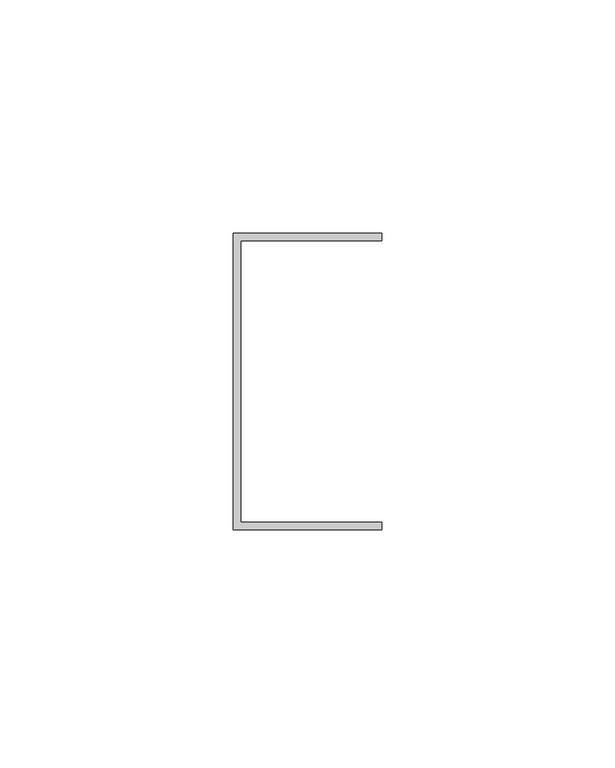
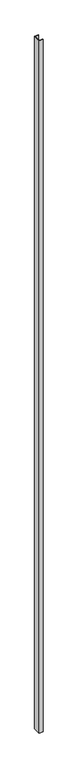
"""IFC4 building model written with IfcOpenShell, lengths in millimetres: proxy geometry, Generic Models 7:Generic Models 1:3:Generic Models 1:3 : Generic Models 7:Generic Models 1:305549:3:Generic Models 1:3:Generic Models 1:3 : Generic Models 7:Generic Models 1:305549:3 : Generic Models 7:Generic Models 1:3:Generic Models 1:3 : Generic Models 7:Generic Models 1:305549:301244:5 : Generic Models 7:Generic Models 1:3:Generic Models 1:3 : Generic Models 7:Generic Models 1:305549:3:Generic Models 1:3:Generic Models 1:3 : Generic Models 7:Generic Models 1:305549:3 : Generic Models 7:Generic Models 1:3:Generic Models 1:3 : Generic Models 7:Generic Models 1:305549:301244:308848."""

from ifc_helpers import new_model, si_unit, frame, origin, place, context, project, spatial, polyline, outline, extrude, source, transform, mapped, element, save


def generic_models_71cab8bc(model_context):
    return source(origin(), model_context, "Body", "SweptSolid", [
        extrude(outline(polyline([(570458.9867239, -579013.3913841), (570490.7367239, -579013.3913841), (570490.7367239, -579014.9788841), (570460.5742239, -579014.9788841), (570460.5742239, -579075.3038841), (570490.7367239, -579075.3038841), (570490.7367239, -579076.8913841), (570458.9867239, -579076.8913841), (570458.9867239, -579013.3913841)])), frame((0.0, 0.0, 38.1), z_axis=(0.0, 0.0, 1.0), x_axis=(1.0, 0.0, 0.0)), (0.0, 0.0, 1.0), 6096.0),
    ])


if __name__ == "__main__":
    model = new_model("IFC4")
    model_context = context("Model", 3, world=origin())
    ifc_project = project(units=[si_unit("LENGTHUNIT", "METRE", prefix="MILLI")], contexts=[model_context])
    site = spatial("IfcSite", under=ifc_project)
    building = spatial("IfcBuilding", under=site)
    placement = place(None, origin())
    generic_models_shape = generic_models_71cab8bc(model_context)
    element("IfcBuildingElementProxy", 1, Name="Generic Models 7:Generic Models 1:3:Generic Models 1:3 : Generic Models 7:Generic Models 1:305549:3:Generic Models 1:3:Generic Models 1:3 : Generic Models 7:Generic Models 1:305549:3 : Generic Models 7:Generic Models 1:3:Generic Models 1:3 : Generic Models 7:Generic Models 1:305549:301244:5 : Generic Models 7:Generic Models 1:3:Generic Models 1:3 : Generic Models 7:Generic Models 1:305549:3:Generic Models 1:3:Generic Models 1:3 : Generic Models 7:Generic Models 1:305549:3 : Generic Models 7:Generic Models 1:3:Generic Models 1:3 : Generic Models 7:Generic Models 1:305549:301244:308848", ObjectType="Generic Models 7:Generic Models 1:3:Generic Models 1:3 : Generic Models 7:Generic Models 1:305549:3:Generic Models 1:3:Generic Models 1:3 : Generic Models 7:Generic Models 1:305549:3 : Generic Models 7:Generic Models 1:3:Generic Models 1:3 : Generic Models 7:Generic Models 1:305549:301244:5 : Generic Models 7:Generic Models 1:3:Generic Models 1:3 : Generic Models 7:Generic Models 1:305549:3:Generic Models 1:3:Generic Models 1:3 : Generic Models 7:Generic Models 1:305549:3 : Generic Models 7:Generic Models 1:3:Generic Models 1:3 : Generic Models 7:Generic Models 1:305549:301244:308848", at=placement, inside=building, context=model_context, shape_type="MappedRepresentation", body=[
        mapped(generic_models_shape, transform((0.0, 0.0, 0.0), x_axis=(1.0, 0.0, 0.0), y_axis=(0.0, 1.0, 0.0), z_axis=(0.0, 0.0, 1.0))),
    ])
    save(model, "model.ifc")

# Revit data of these elements
# Type "Generic Models 7:Generic Models 1:3:Generic Models 1:3 : Generic Models 7:Generic Models 1:305549:3:Generic Models 1:3:Generic Models 1:3 : Generic Models 7:Generic Models 1:305549:3 : Generic Models 7:Generic Models 1:3:Generic Models 1:3 : Generic Models 7:Generic Models 1:305549:301244:5 : Generic Models 7:Generic Models 1:3:Generic Models 1:3 : Generic Models 7:Generic Models 1:305549:3:Generic Models 1:3:Generic Models 1:3 : Generic Models 7:Generic Models 1:305549:3 : Generic Models 7:Generic Models 1:3:Generic Models 1:3 : Generic Models 7:Generic Models 1:305549:301244:308848"
#   NameOverride = "Generic Models 7:Generic Models 1:3:Generic Models 1:3 : Generic Models 7:Generic Models 1:305549:3:Generic Models 1:3:Generic Models 1:3 : Generic Models 7:Generic Models 1:305549:3 : Generic Models 7:Generic Models 1:3:Generic Models 1:3 : Generic Models 7:Generic Models 1:305549:301244:308848"
#   ObjectTypeOverride = "Generic Models 1:3:Generic Models 1:3 : Generic Models 7:Generic Models 1:305549:3 : Generic Models 7:Generic Models 1:3:Generic Models 1:3 : Generic Models 7:Generic Models 1:305549:301244"
#   Reference = "Generic Models 1"
#   Tag = "308848"
# Element 1 (IfcBuildingElementProxy, "Generic Models 7:Generic Models 1:3:Generic Models 1:3 : Generic Models 7:Generic Models 1:305549:3:Generic Models 1:3:Generic Models 1:3 : Generic Models 7:Generic Models 1:305549:3 : Generic Models 7:Generic Models 1:3:Generic Models 1:3 : Generic Models 7:Generic Models 1:305549:301244:5 : Generic Models 7:Generic Models 1:3:Generic Models 1:3 : Generic Models 7:Generic Models 1:305549:3:Generic Models 1:3:Generic Models 1:3 : Generic Models 7:Generic Models 1:305549:3 : Generic Models 7:Generic Models 1:3:Generic Models 1:3 : Generic Models 7:Generic Models 1:305549:301244:308848")
#   Materials on its faces: "GALVANIZED U-CHANNEL (250T125-33)"
# Materials
#   "GALVANIZED U-CHANNEL (250T125-33)": class "Unassigned", colour RGB 202 201 200, transparency 0, Keynote = "M05451300.02", Cost = 0
